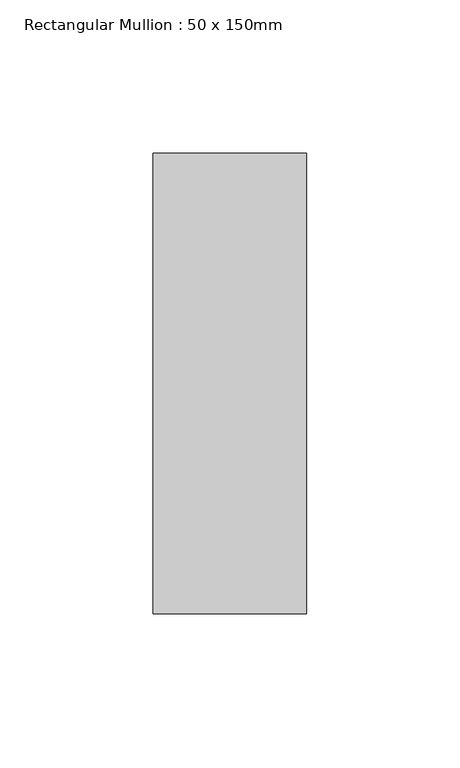
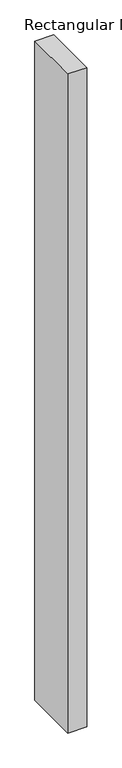
"""IFC4 building model written with IfcOpenShell, lengths in millimetres: member geometry, Rectangular Mullion : 50 x 150mm."""

from ifc_helpers import new_model, si_unit, frame, origin, place, context, project, spatial, polyline, outline, extrude, source, transform, mapped, element, save


def rectangular_mullion_50_x_150mm_e08e94d7(model_context):
    return source(origin(), model_context, "Body", "SweptSolid", [
        extrude(outline(polyline([(0.0, 75.0), (0.0, -75.0), (-50.0, -75.0), (-50.0, 75.0), (0.0, 75.0)])), frame((0.0, 0.0, -1838.8888888), z_axis=(0.0, 0.0, 1.0), x_axis=(1.0, 0.0, 0.0)), (0.0, 0.0, 1.0), 1838.8888888),
    ])


if __name__ == "__main__":
    model = new_model("IFC4")
    model_context = context("Model", 3, world=origin())
    ifc_project = project(units=[si_unit("LENGTHUNIT", "METRE", prefix="MILLI")], contexts=[model_context])
    site = spatial("IfcSite", under=ifc_project)
    building = spatial("IfcBuilding", under=site)
    placement = place(None, origin())
    rectangular_mullion_50_x_150mm_shape = rectangular_mullion_50_x_150mm_e08e94d7(model_context)
    element("IfcMember", 1, ObjectType="Rectangular Mullion : 50 x 150mm", at=placement, inside=building, context=model_context, shape_type="MappedRepresentation", body=[
        mapped(rectangular_mullion_50_x_150mm_shape, transform((0.0, 0.0, 0.0), x_axis=(1.0, 0.0, 0.0), y_axis=(0.0, 1.0, 0.0), z_axis=(0.0, 0.0, 1.0))),
    ])
    save(model, "model.ifc")

# Revit data of these elements
# Type "Rectangular Mullion : 50 x 150mm"
#   built-in parameter 1007304 = 0.492126 (stored number, unit not read)
#   built-in parameter 1007301 = 0.082021 (stored number, unit not read)
#   built-in parameter 1007300 = 0.082021 (stored number, unit not read)
# Element 1 (IfcMember, "Rectangular Mullion : 50 x 150mm")
#   Materials on its faces: "Metal - Aluminium"
# Materials
#   "Metal - Aluminium": class "Metal", colour RGB 247 247 247, transparency 0
